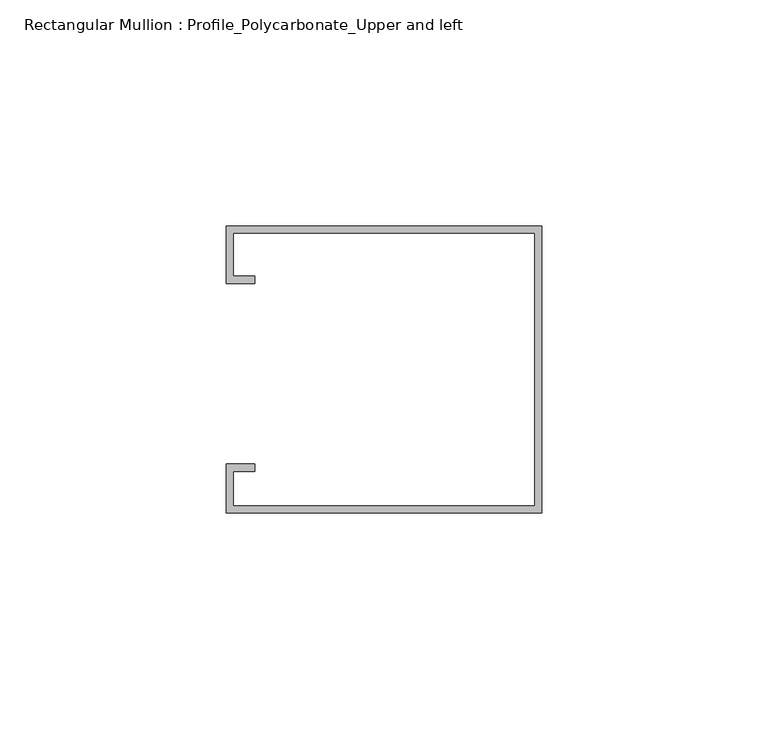
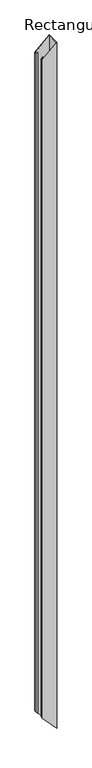
"""IFC4 building model written with IfcOpenShell, lengths in millimetres: member geometry, Rectangular Mullion : Profile_Polycarbonate_Upper and left."""

from ifc_helpers import new_model, si_unit, origin, place, context, project, spatial, faceted_brep, source, transform, mapped, element, save


def rectangular_mullion_profile_polycarbonate_upper_and_left_966177da(model_context):
    return source(origin(), model_context, "Body", "Brep", [
        faceted_brep([(-69.85, 32.7, -64.2712818), (0.0, 32.7, 0.0), (0.0, 32.7, -3503.0127529), (-69.85, 32.7, -3427.0998045), (-69.85, 20.0, -64.2712818), (-69.85, 20.0, -3427.0998045), (-63.5, 20.0, -58.428438), (-63.5, 20.0, -3434.0009816), (-63.5, 21.5875, -58.428438), (-63.5, 21.5875, -3434.0009816), (-68.2625, 21.5875, -62.8105708), (-68.2625, 21.5875, -3428.8250988), (-68.2625, 31.1125, -62.8105708), (-68.2625, 31.1125, -3428.8250988), (-1.5875, 31.1125, -1.4607109), (-1.5875, 31.1125, -3501.2874586), (-1.5875, -29.2125, -1.4607109), (-1.5875, -29.2125, -3501.2874586), (-68.2625, -29.2125, -62.8105708), (-68.2625, -29.2125, -3428.8250988), (-68.2625, -21.5875, -62.8105708), (-68.2625, -21.5875, -3428.8250988), (-63.5, -21.5875, -58.428438), (-63.5, -21.5875, -3434.0009816), (-63.5, -20.0, -58.428438), (-63.5, -20.0, -3434.0009816), (-69.85, -20.0, -64.2712818), (-69.85, -20.0, -3427.0998045), (-69.85, -30.8, -64.2712818), (-69.85, -30.8, -3427.0998045), (0.0, -30.8, 0.0), (0.0, -30.8, -3503.0127529)], [[[0, 1, 2, 3]], [[4, 0, 3, 5]], [[6, 4, 5, 7]], [[8, 6, 7, 9]], [[10, 8, 9, 11]], [[12, 10, 11, 13]], [[14, 12, 13, 15]], [[16, 14, 15, 17]], [[18, 16, 17, 19]], [[20, 18, 19, 21]], [[22, 20, 21, 23]], [[24, 22, 23, 25]], [[26, 24, 25, 27]], [[28, 26, 27, 29]], [[30, 28, 29, 31]], [[1, 30, 31, 2]], [[1, 0, 4, 6, 8, 10, 12, 14, 16, 18, 20, 22, 24, 26, 28, 30]], [[2, 31, 29, 27, 25, 23, 21, 19, 17, 15, 13, 11, 9, 7, 5, 3]]]),
    ])


if __name__ == "__main__":
    model = new_model("IFC4")
    model_context = context("Model", 3, world=origin())
    ifc_project = project(units=[si_unit("LENGTHUNIT", "METRE", prefix="MILLI")], contexts=[model_context])
    site = spatial("IfcSite", under=ifc_project)
    building = spatial("IfcBuilding", under=site)
    placement = place(None, origin())
    rectangular_mullion_profile_polycarbonate_upper_and_left_shape = rectangular_mullion_profile_polycarbonate_upper_and_left_966177da(model_context)
    element("IfcMember", 1, ObjectType="Rectangular Mullion : Profile_Polycarbonate_Upper and left", at=placement, inside=building, context=model_context, shape_type="MappedRepresentation", body=[
        mapped(rectangular_mullion_profile_polycarbonate_upper_and_left_shape, transform((0.0, 0.0, 0.0), x_axis=(1.0, 0.0, 0.0), y_axis=(0.0, 1.0, 0.0), z_axis=(0.0, 0.0, 1.0))),
    ])
    save(model, "model.ifc")

# Revit data of these elements
# Type "Rectangular Mullion : Profile_Polycarbonate_Upper and left"
#   built-in parameter 1007322 = 0.208333 (stored number, unit not read)
#   built-in parameter 1007321 = 0.00520833 (stored number, unit not read)
#   built-in parameter 1007320 = 0 (stored number, unit not read)
# Element 1 (IfcMember, "Rectangular Mullion : Profile_Polycarbonate_Upper and left")
#   Materials on its faces: "ALUMINUM PROFILE AT POLYCARBONATE PANEL"
# Materials
#   "ALUMINUM PROFILE AT POLYCARBONATE PANEL": class "Metal", colour RGB 244 244 244, transparency 0, Description = "Aluminum 6061", Cost = 0
